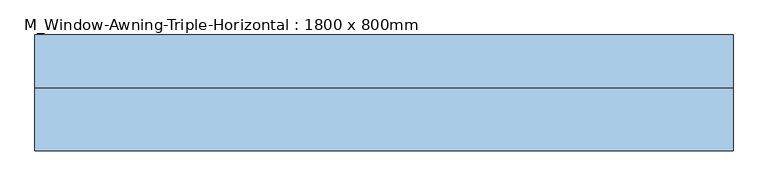
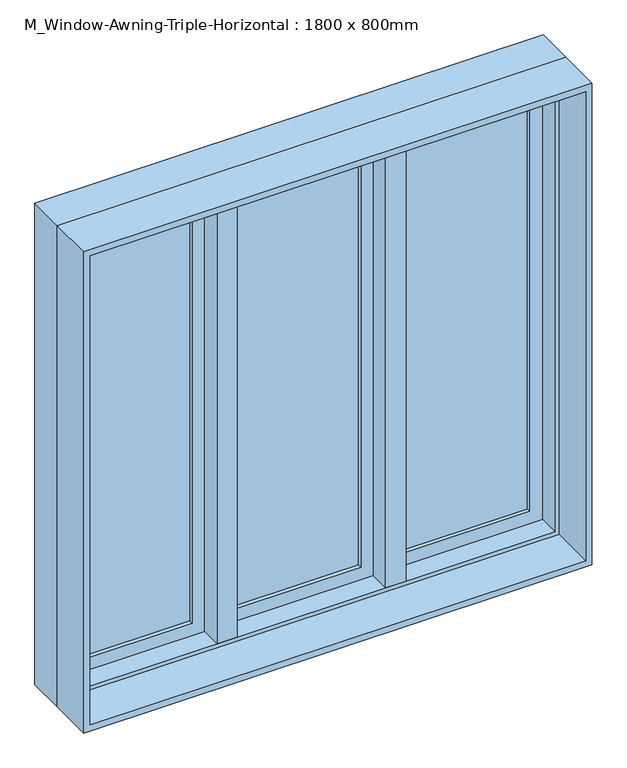
"""IFC4 building model written with IfcOpenShell, lengths in millimetres: window geometry, M_Window-Awning-Triple-Horizontal : 1800 x 800mm."""

from ifc_helpers import new_model, si_unit, frame, origin, place, context, project, spatial, polyline, outline, extrude, faceted_brep, source, transform, mapped, element, save


def m_window_awning_triple_horizontal_1800_x_800mm_57cedfb2(model_context):
    return source(origin(), model_context, "Body", "SolidModel", [
        faceted_brep([(239.4166667, 83.25, 2387.3), (218.9065328, 83.25, 2387.3), (218.9065328, 19.75, 2387.3), (278.9768005, 19.75, 2387.3), (278.9768005, 83.25, 2387.3), (258.4666667, 83.25, 2387.3), (258.4666667, 134.05, 2387.3), (239.4166667, 134.05, 2387.3), (239.4166667, 134.05, 912.7), (258.4666667, 134.05, 912.7), (258.4666667, 105.475, 912.7), (239.4166667, 105.475, 912.7), (239.4166667, 83.25, 2380.95), (218.9065328, 83.25, 2380.95), (239.4166667, 83.25, 2368.25), (239.4166667, 83.25, 931.75), (218.9065328, 83.25, 931.75), (218.9065328, 83.25, 2368.25), (218.9065328, 19.75, 2380.95), (218.9065328, 19.75, 931.75), (218.9065328, 19.75, 2368.25), (278.9768005, 19.75, 2380.95), (278.9768005, 19.75, 931.75), (278.9768005, 19.75, 2368.25), (278.9768005, 83.25, 2380.95), (278.9768005, 83.25, 931.75), (278.9768005, 83.25, 2368.25), (258.4666667, 83.25, 2380.95), (258.4666667, 83.25, 931.75), (258.4666667, 83.25, 2368.25), (258.4666667, 105.475, 2380.95), (258.4666667, 105.475, 2368.25), (258.4666667, 105.475, 931.75), (239.4166667, 105.475, 931.75), (239.4166667, 105.475, 2368.25), (239.4166667, 105.475, 2380.95)], [[[0, 1, 2, 3, 4, 5, 6, 7]], [[8, 9, 10, 11]], [[1, 0, 12, 13]], [[14, 15, 16, 17]], [[2, 1, 13, 18]], [[17, 16, 19, 20]], [[3, 2, 18, 21]], [[20, 19, 22, 23]], [[4, 3, 21, 24]], [[23, 22, 25, 26]], [[5, 4, 24, 27]], [[26, 25, 28, 29]], [[6, 5, 27, 30, 31, 29, 28, 32, 10, 9]], [[0, 7, 8, 11, 33, 15, 14, 34, 35, 12]], [[30, 35, 34, 31]], [[32, 33, 11, 10]], [[35, 30, 27, 24, 21, 18, 13, 12]], [[31, 34, 14, 17, 20, 23, 26, 29]], [[33, 32, 28, 25, 22, 19, 16, 15]], [[7, 6, 9, 8]]]),
        faceted_brep([(-258.4666667, 83.25, 2387.3), (-278.9768005, 83.25, 2387.3), (-278.9768005, 19.75, 2387.3), (-218.9065328, 19.75, 2387.3), (-218.9065328, 83.25, 2387.3), (-239.4166667, 83.25, 2387.3), (-239.4166667, 134.05, 2387.3), (-258.4666667, 134.05, 2387.3), (-258.4666667, 134.05, 912.7), (-239.4166667, 134.05, 912.7), (-239.4166667, 105.475, 912.7), (-258.4666667, 105.475, 912.7), (-278.9768005, 83.25, 2380.95), (-278.9768005, 19.75, 2380.95), (-278.9768005, 83.25, 2368.25), (-278.9768005, 83.25, 931.75), (-278.9768005, 19.75, 931.75), (-278.9768005, 19.75, 2368.25), (-218.9065328, 19.75, 2380.95), (-218.9065328, 19.75, 931.75), (-218.9065328, 19.75, 2368.25), (-218.9065328, 83.25, 2380.95), (-218.9065328, 83.25, 931.75), (-218.9065328, 83.25, 2368.25), (-239.4166667, 83.25, 2380.95), (-239.4166667, 105.475, 2380.95), (-239.4166667, 105.475, 2368.25), (-239.4166667, 83.25, 2368.25), (-239.4166667, 83.25, 931.75), (-239.4166667, 105.475, 931.75), (-258.4666667, 105.475, 931.75), (-258.4666667, 83.25, 931.75), (-258.4666667, 83.25, 2368.25), (-258.4666667, 105.475, 2368.25), (-258.4666667, 105.475, 2380.95), (-258.4666667, 83.25, 2380.95)], [[[0, 1, 2, 3, 4, 5, 6, 7]], [[8, 9, 10, 11]], [[2, 1, 12, 13]], [[14, 15, 16, 17]], [[3, 2, 13, 18]], [[17, 16, 19, 20]], [[4, 3, 18, 21]], [[20, 19, 22, 23]], [[6, 5, 24, 25, 26, 27, 28, 29, 10, 9]], [[0, 7, 8, 11, 30, 31, 32, 33, 34, 35]], [[25, 34, 33, 26]], [[29, 30, 11, 10]], [[34, 25, 24, 21, 18, 13, 12, 35]], [[26, 33, 32, 14, 17, 20, 23, 27]], [[30, 29, 28, 22, 19, 16, 15, 31]], [[1, 0, 35, 12]], [[15, 14, 32, 31]], [[5, 4, 21, 24]], [[28, 27, 23, 22]], [[7, 6, 9, 8]]]),
        extrude(outline(polyline([(912.7, 239.4166667), (2387.3, 239.4166667), (2387.3, -239.4166667), (912.7, -239.4166667), (912.7, 239.4166667)]), holes=[polyline([(969.85, -182.2666667), (2330.15, -182.2666667), (2330.15, 182.2666667), (969.85, 182.2666667), (969.85, -182.2666667)])]), frame((0.0, 83.25, 0.0), z_axis=(0.0, 1.0, 0.0), x_axis=(0.0, 0.0, 1.0)), (0.0, 0.0, 1.0), 44.45),
        extrude(outline(polyline([(182.2666667, 115.0), (182.2666667, 108.65), (-182.2666667, 108.65), (-182.2666667, 115.0), (182.2666667, 115.0)])), frame((0.0, 0.0, 969.85), z_axis=(0.0, 0.0, 1.0), x_axis=(1.0, 0.0, 0.0)), (0.0, 0.0, 1.0), 1360.3),
        extrude(outline(polyline([(-182.2666667, 95.95), (-182.2666667, 102.3), (182.2666667, 102.3), (182.2666667, 95.95), (-182.2666667, 95.95)])), frame((0.0, 0.0, 969.85), z_axis=(0.0, 0.0, 1.0), x_axis=(1.0, 0.0, 0.0)), (0.0, 0.0, 1.0), 1360.3),
        extrude(outline(polyline([(-315.6166667, 115.0), (-315.6166667, 108.65), (-680.15, 108.65), (-680.15, 115.0), (-315.6166667, 115.0)])), frame((0.0, 0.0, 969.85), z_axis=(0.0, 0.0, 1.0), x_axis=(1.0, 0.0, 0.0)), (0.0, 0.0, 1.0), 1360.3),
        extrude(outline(polyline([(-680.15, 95.95), (-680.15, 102.3), (-315.6166667, 102.3), (-315.6166667, 95.95), (-680.15, 95.95)])), frame((0.0, 0.0, 969.85), z_axis=(0.0, 0.0, 1.0), x_axis=(1.0, 0.0, 0.0)), (0.0, 0.0, 1.0), 1360.3),
        extrude(outline(polyline([(680.15, 115.0), (680.15, 108.65), (315.6166667, 108.65), (315.6166667, 115.0), (680.15, 115.0)])), frame((0.0, 0.0, 969.85), z_axis=(0.0, 0.0, 1.0), x_axis=(1.0, 0.0, 0.0)), (0.0, 0.0, 1.0), 1360.3),
        extrude(outline(polyline([(315.6166667, 95.95), (315.6166667, 102.3), (680.15, 102.3), (680.15, 95.95), (315.6166667, 95.95)])), frame((0.0, 0.0, 969.85), z_axis=(0.0, 0.0, 1.0), x_axis=(1.0, 0.0, 0.0)), (0.0, 0.0, 1.0), 1360.3),
        extrude(outline(polyline([(2387.3, -737.3), (912.7, -737.3), (912.7, -258.4666667), (2387.3, -258.4666667), (2387.3, -737.3)]), holes=[polyline([(2330.15, -315.6166667), (969.85, -315.6166667), (969.85, -680.15), (2330.15, -680.15), (2330.15, -315.6166667)])]), frame((0.0, 83.25, 0.0), z_axis=(0.0, 1.0, 0.0), x_axis=(0.0, 0.0, 1.0)), (0.0, 0.0, 1.0), 44.45),
        extrude(outline(polyline([(912.7, 737.3), (2387.3, 737.3), (2387.3, 258.4666667), (912.7, 258.4666667), (912.7, 737.3)]), holes=[polyline([(969.85, 315.6166667), (2330.15, 315.6166667), (2330.15, 680.15), (969.85, 680.15), (969.85, 315.6166667)])]), frame((0.0, 83.25, 0.0), z_axis=(0.0, 1.0, 0.0), x_axis=(0.0, 0.0, 1.0)), (0.0, 0.0, 1.0), 44.45),
        extrude(outline(polyline([(2400.0, -750.0), (900.0, -750.0), (900.0, 750.0), (2400.0, 750.0), (2400.0, -750.0)]), holes=[polyline([(2380.95, 730.95), (919.05, 730.95), (919.05, -730.95), (2380.95, -730.95), (2380.95, 730.95)])]), frame((0.0, -115.0, 0.0), z_axis=(0.0, 1.0, 0.0), x_axis=(0.0, 0.0, 1.0)), (0.0, 0.0, 1.0), 134.75),
        faceted_brep([(718.25, 83.25, 2368.25), (718.25, 19.75, 2368.25), (-718.25, 19.75, 2368.25), (-718.25, 83.25, 2368.25), (737.3, 134.05, 2387.3), (737.3, 83.25, 2387.3), (-737.3, 83.25, 2387.3), (-737.3, 134.05, 2387.3), (750.0, 19.75, 2400.0), (750.0, 134.05, 2400.0), (-750.0, 134.05, 2400.0), (-750.0, 19.75, 2400.0), (-718.25, 19.75, 931.75), (-718.25, 83.25, 931.75), (-737.3, 83.25, 912.7), (-737.3, 134.05, 912.7), (-750.0, 134.05, 900.0), (-750.0, 19.75, 900.0), (718.25, 19.75, 931.75), (718.25, 83.25, 931.75), (737.3, 83.25, 912.7), (737.3, 134.05, 912.7), (750.0, 134.05, 900.0), (750.0, 19.75, 900.0)], [[[0, 1, 2, 3]], [[4, 5, 6, 7]], [[8, 9, 10, 11]], [[3, 2, 12, 13]], [[7, 6, 14, 15]], [[11, 10, 16, 17]], [[13, 12, 18, 19]], [[15, 14, 20, 21]], [[17, 16, 22, 23]], [[11, 17, 23, 8], [1, 18, 12, 2]], [[19, 18, 1, 0]], [[5, 20, 14, 6], [3, 13, 19, 0]], [[21, 20, 5, 4]], [[23, 22, 9, 8]], [[9, 22, 16, 10], [7, 15, 21, 4]]]),
    ])


if __name__ == "__main__":
    model = new_model("IFC4")
    model_context = context("Model", 3, world=origin())
    ifc_project = project(units=[si_unit("LENGTHUNIT", "METRE", prefix="MILLI")], contexts=[model_context])
    site = spatial("IfcSite", under=ifc_project)
    building = spatial("IfcBuilding", under=site)
    placement = place(None, origin())
    m_window_awning_triple_horizontal_1800_x_800mm_shape = m_window_awning_triple_horizontal_1800_x_800mm_57cedfb2(model_context)
    element("IfcWindow", 1, ObjectType="M_Window-Awning-Triple-Horizontal : 1800 x 800mm", at=placement, inside=building, context=model_context, shape_type="MappedRepresentation", body=[
        mapped(m_window_awning_triple_horizontal_1800_x_800mm_shape, transform((0.0, 0.0, 0.0), x_axis=(1.0, 0.0, 0.0), y_axis=(0.0, 1.0, 0.0), z_axis=(0.0, 0.0, 1.0))),
    ])
    save(model, "model.ifc")

# Revit data of these elements
# Type "M_Window-Awning-Triple-Horizontal : 1800 x 800mm"
#   Type Mark = "39"
#   Fire Rating = "0.5h"
#   Assembly Code = "B2020100"
#   Analytic Construction = "Double glazing - domestic"
#   Window Inset [instance default] = 0 m
#   Wall Thickness [instance default] = 0.15 m
#   Muntin Width = 0.364533 m
#   Visual Light Transmittance = 0.81
#   Thermal Resistance (R) = 0.319569 (m²·K)/W
#   Solar Heat Gain Coefficient = 0.76
#   One Third Width = 0.5 m
#   Sash Width = 0.478833 m
#   Rough Width = 1.515 m
#   Rough Height = 1.515 m
#   Interior Wall Closure [instance default] = 0.05475 m
#   Height = 1.5 m
#   Heat Transfer Coefficient (U) = 3.12929 W/(m²·K)
#   Muntin Height = 1.3603 m
#   Frame Extension [instance default] = 0.00635 m
#   Exterior Wall Closure [instance default] = 0.03175 m
#   Extension Jamb [instance default] = 0.05475 m
#   Default Sill Height = 0.9 m
#   Width = 1.5 m
#   Middle Muntin Visibility = yes
#   Side Muntin Visibility = yes
#   Interior Trim Visibility [instance default] = yes
#   Exterior Trim Visibility [instance default] = yes
#   Extension Jamb Visibility [instance default] = yes
#   Muntin Pattern = M_Muntin Pattern_2x2 : M_Muntin Pattern_2x2
#   Interior Trim Material = Wood - Stained
#   Interior Trim = M_Trim-Window-Interior-Flat : Picture Frame
#   Interior Frame Material = Wood - Stained
#   Glass Panel Material = Glass
#   Exterior Trim Material = Clad - White
#   Exterior Trim = M_Trim-Window-Exterior-Flat : with Sill
#   Exterior Frame Material = Clad - White
#   Wall Closure = (empty or 0)
# Element 1 (IfcWindow, "M_Window-Awning-Triple-Horizontal : 1800 x 800mm")
#   Wall Thickness = 0.23 m
#   Extension Jamb = 0.13475 m
#   Materials on its faces: "Wood - Stained", "Glass", "Clad - White"
# Materials
#   "Wood - Stained": class "Wood", colour RGB 224 178 126, transparency 0, Cost = 0
#   "Glass": class "Glass", colour RGB 0 128 192, transparency 0.9, Description = "Soda Lime Glass", Cost = 0
#   "Clad - White": class "Wood", colour RGB 242 242 238, transparency 0, Cost = 0
